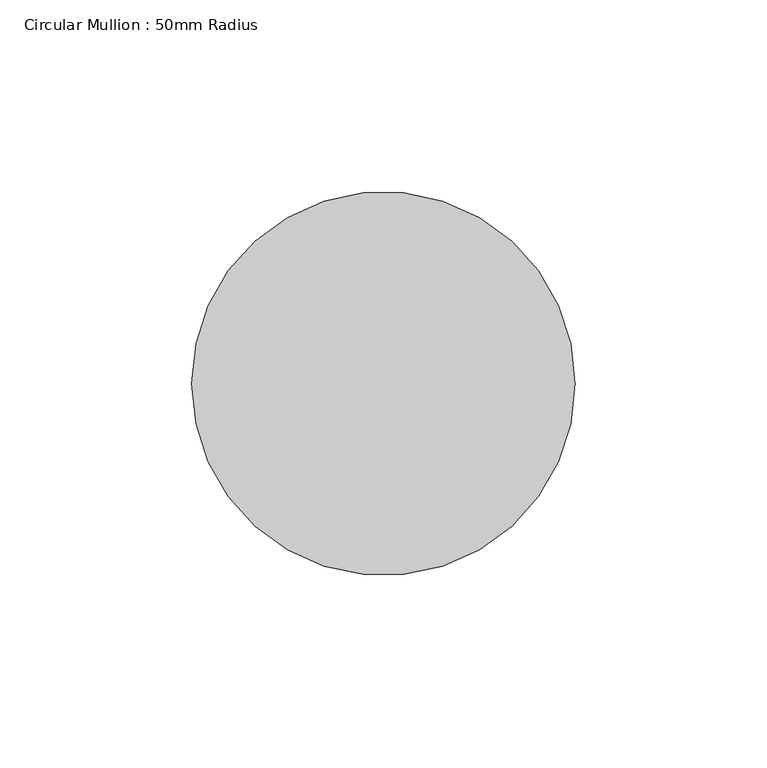
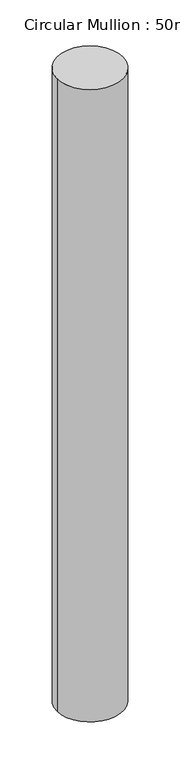
"""IFC4 building model written with IfcOpenShell, lengths in millimetres: member geometry, Circular Mullion : 50mm Radius."""

from ifc_helpers import new_model, si_unit, point, frame, origin, origin_2d, place, context, project, spatial, circle_curve, trimmed, segment, composite_curve, outline, extrude, source, transform, mapped, element, save


def circular_mullion_50mm_radius_cb04586f(model_context):
    return source(origin(), model_context, "Body", "SweptSolid", [
        extrude(outline(composite_curve([segment(trimmed(circle_curve(origin_2d(), 50.0), [point((50.0, 0.0))], [point((-50.0, 0.0))], False, "CARTESIAN"), True, "CONTINUOUS"), segment(trimmed(circle_curve(origin_2d(), 50.0), [point((-50.0, 0.0))], [point((50.0, 0.0))], False, "CARTESIAN"), True, "CONTINUOUS")], self_intersect=False)), frame((0.0, 0.0, -1015.6228811), z_axis=(0.0, 0.0, 1.0), x_axis=(1.0, 0.0, 0.0)), (0.0, 0.0, 1.0), 1015.6228811),
    ])


if __name__ == "__main__":
    model = new_model("IFC4")
    model_context = context("Model", 3, world=origin())
    ifc_project = project(units=[si_unit("LENGTHUNIT", "METRE", prefix="MILLI")], contexts=[model_context])
    site = spatial("IfcSite", under=ifc_project)
    building = spatial("IfcBuilding", under=site)
    placement = place(None, origin())
    circular_mullion_50mm_radius_shape = circular_mullion_50mm_radius_cb04586f(model_context)
    element("IfcMember", 1, ObjectType="Circular Mullion : 50mm Radius", at=placement, inside=building, context=model_context, shape_type="MappedRepresentation", body=[
        mapped(circular_mullion_50mm_radius_shape, transform((0.0, 0.0, 0.0), x_axis=(1.0, 0.0, 0.0), y_axis=(0.0, 1.0, 0.0), z_axis=(0.0, 0.0, 1.0))),
    ])
    save(model, "model.ifc")

# Revit data of these elements
# Type "Circular Mullion : 50mm Radius"
#   built-in parameter 1007350 = 0.164042 (stored number, unit not read)
# Element 1 (IfcMember, "Circular Mullion : 50mm Radius")
#   Materials on its faces: "Aluminium"
# Materials
#   "Aluminium": class "Metal", colour RGB 247 247 247, transparency 0, Description = "Aluminium 6061", Cost = 0
